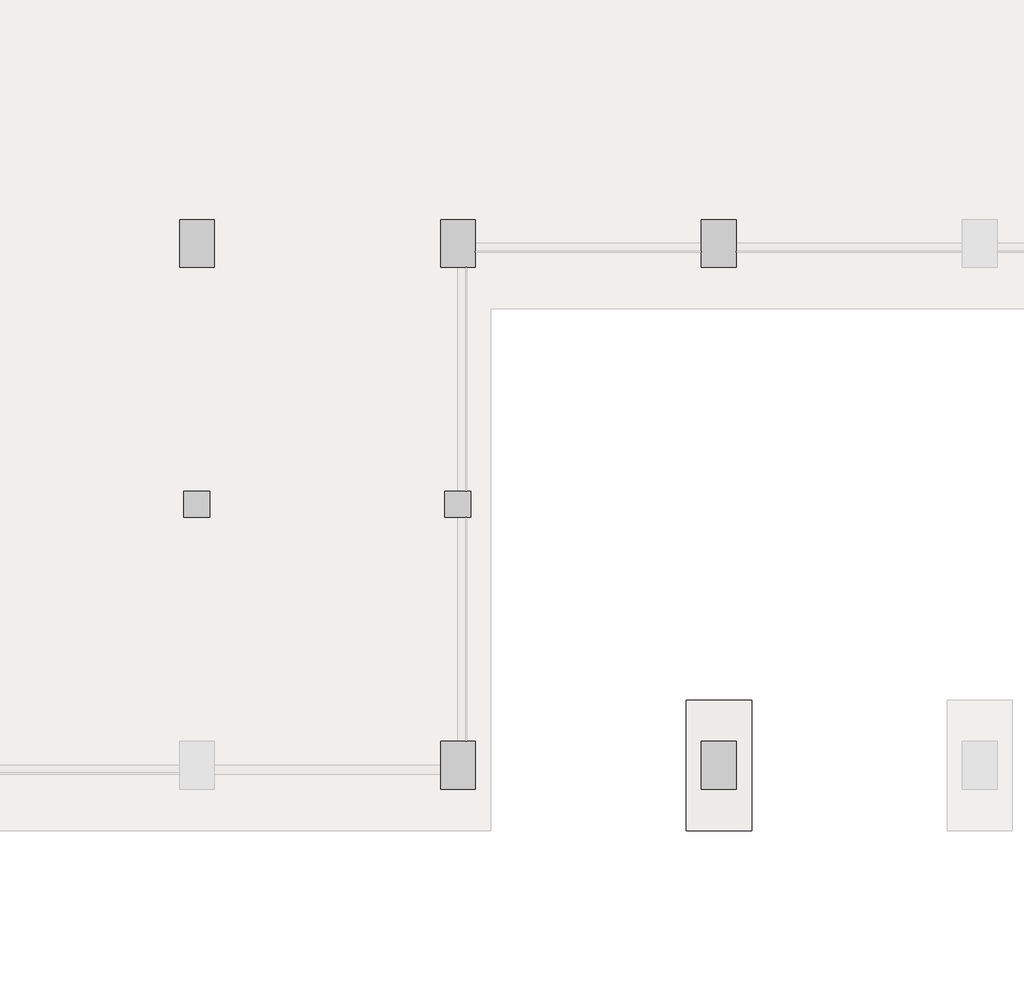
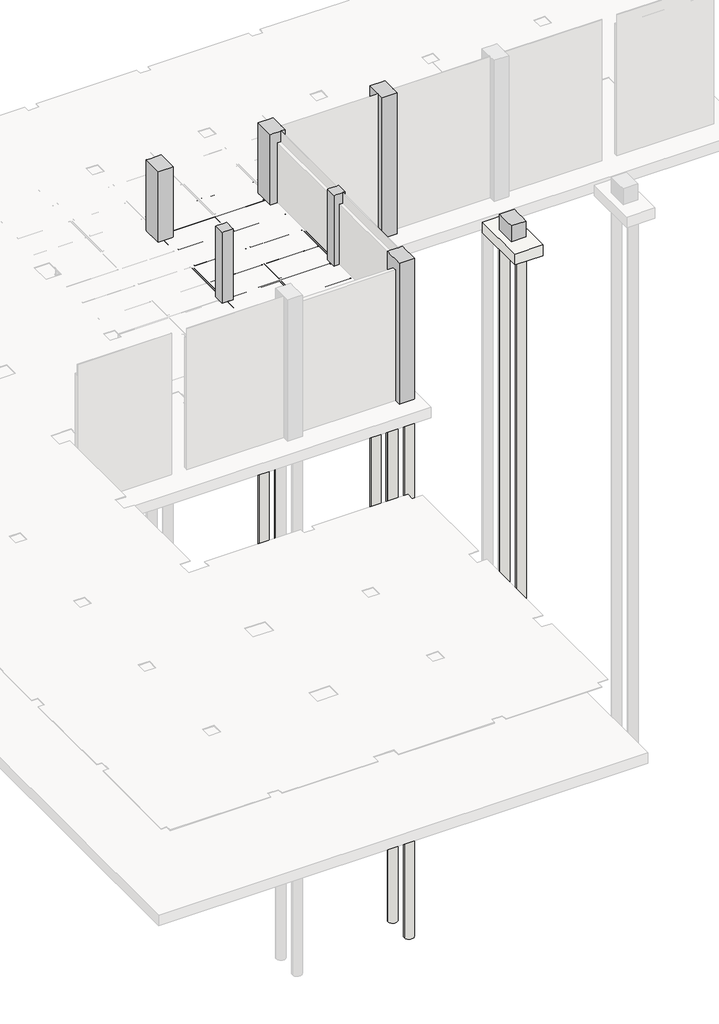
# Not in any storey, part 11 of 16: 24 beams, 9 slabs, 7 columns.
"""IFC4 building model written with IfcOpenShell, lengths in millimetres."""

from ifc_helpers import new_model, si_unit, point, frame, frame_2d, origin, place, context, project, spatial, polyline, circle_curve, trimmed, segment, composite_curve, outline, extrude, faceted_brep, element, save

model = new_model("IFC4")

# Units and contexts
model_context = context("Model", 3, world=origin())
ifc_project = project(units=[si_unit("LENGTHUNIT", "METRE", prefix="MILLI")], contexts=[model_context])

# Site, building
site = spatial("IfcSite", under=ifc_project)
building = spatial("IfcBuilding", under=site)

# Beams
placement = place(None, origin())
element("IfcBeam", 1, ObjectType="Steel Framing_H_KS : H_SB_AR_S02_H-400x200x8x13_BSG1", at=placement, inside=building, context=model_context, shape_type="SweptSolid", body=[
    extrude(outline(composite_curve([segment(polyline([(-17900.0, -4187.0381366), (-17900.0, -4200.0381366), (-18100.0, -4200.0381366), (-18100.0, -4187.0381366), (-18020.0, -4187.0381366)]), True, "CONTINUOUS"), segment(trimmed(circle_curve(frame_2d((-18020.0, -4171.0381366)), 16.0), [point((-18020.0, -4187.0381366))], [point((-18004.0, -4171.0381366))], True, "CARTESIAN"), True, "CONTINUOUS"), segment(polyline([(-18004.0, -4171.0381366), (-18004.0, -3829.0381366)]), True, "CONTINUOUS"), segment(trimmed(circle_curve(frame_2d((-18020.0, -3829.0381366)), 16.0), [point((-18004.0, -3829.0381366))], [point((-18020.0, -3813.0381366))], True, "CARTESIAN"), True, "CONTINUOUS"), segment(polyline([(-18020.0, -3813.0381366), (-18100.0, -3813.0381366), (-18100.0, -3800.0381366), (-17900.0, -3800.0381366), (-17900.0, -3813.0381366), (-17980.0, -3813.0381366)]), True, "CONTINUOUS"), segment(trimmed(circle_curve(frame_2d((-17980.0, -3829.0381366)), 16.0), [point((-17980.0, -3813.0381366))], [point((-17996.0, -3829.0381366))], True, "CARTESIAN"), True, "CONTINUOUS"), segment(polyline([(-17996.0, -3829.0381366), (-17996.0, -4171.0381366)]), True, "CONTINUOUS"), segment(trimmed(circle_curve(frame_2d((-17980.0, -4171.0381366)), 16.0), [point((-17996.0, -4171.0381366))], [point((-17980.0, -4187.0381366))], True, "CARTESIAN"), True, "CONTINUOUS"), segment(polyline([(-17980.0, -4187.0381366), (-17900.0, -4187.0381366)]), True, "CONTINUOUS")], self_intersect=False)), frame((48412.7, 0.0, 0.0), z_axis=(1.0, 0.0, 0.0), x_axis=(0.0, 1.0, 0.0)), (0.0, 0.0, 1.0), 5174.6),
])
element("IfcBeam", 2, ObjectType="Steel Framing_C_KS : H_SB_AR_S02_C-150x75x6.5x10_J1", at=placement, inside=building, context=model_context, shape_type="SweptSolid", body=[
    extrude(outline(composite_curve([segment(polyline([(-16477.2, -3800.0381366), (-16477.2, -3950.0381366), (-16552.2, -3950.0381366)]), True, "CONTINUOUS"), segment(trimmed(circle_curve(frame_2d((-16542.2, -3950.0381366)), 10.0), [point((-16552.2, -3950.0381366))], [point((-16542.2, -3940.0381366))], False, "CARTESIAN"), True, "CONTINUOUS"), segment(polyline([(-16542.2, -3940.0381366), (-16483.7, -3930.7726469), (-16483.7, -3819.3036264), (-16542.2, -3810.0381366)]), True, "CONTINUOUS"), segment(trimmed(circle_curve(frame_2d((-16542.2, -3800.0381366)), 10.0), [point((-16542.2, -3810.0381366))], [point((-16552.2, -3800.0381366))], False, "CARTESIAN"), True, "CONTINUOUS"), segment(polyline([(-16552.2, -3800.0381366), (-16477.2, -3800.0381366)]), True, "CONTINUOUS")], self_intersect=False)), frame((48112.7, 0.0, 0.0), z_axis=(1.0, 0.0, 0.0), x_axis=(0.0, 1.0, 0.0)), (0.0, 0.0, 1.0), 2774.6),
])
element("IfcBeam", 3, ObjectType="Steel Framing_C_KS : H_SB_AR_S02_C-150x75x6.5x10_J1", at=placement, inside=building, context=model_context, shape_type="SweptSolid", body=[
    extrude(outline(composite_curve([segment(polyline([(-16477.2, -3800.0381366), (-16477.2, -3950.0381366), (-16552.2, -3950.0381366)]), True, "CONTINUOUS"), segment(trimmed(circle_curve(frame_2d((-16542.2, -3950.0381366)), 10.0), [point((-16552.2, -3950.0381366))], [point((-16542.2, -3940.0381366))], False, "CARTESIAN"), True, "CONTINUOUS"), segment(polyline([(-16542.2, -3940.0381366), (-16483.7, -3930.7726469), (-16483.7, -3819.3036264), (-16542.2, -3810.0381366)]), True, "CONTINUOUS"), segment(trimmed(circle_curve(frame_2d((-16542.2, -3800.0381366)), 10.0), [point((-16542.2, -3810.0381366))], [point((-16552.2, -3800.0381366))], False, "CARTESIAN"), True, "CONTINUOUS"), segment(polyline([(-16552.2, -3800.0381366), (-16477.2, -3800.0381366)]), True, "CONTINUOUS")], self_intersect=False)), frame((51112.7, 0.0, 0.0), z_axis=(1.0, 0.0, 0.0), x_axis=(0.0, 1.0, 0.0)), (0.0, 0.0, 1.0), 2774.6),
])
element("IfcBeam", 4, ObjectType="Steel Framing_C_KS : H_SB_AR_S02_C-150x75x6.5x10_J1", at=placement, inside=building, context=model_context, shape_type="SweptSolid", body=[
    extrude(outline(composite_curve([segment(polyline([(-16477.2, -3800.0381366), (-16477.2, -3950.0381366), (-16552.2, -3950.0381366)]), True, "CONTINUOUS"), segment(trimmed(circle_curve(frame_2d((-16542.2, -3950.0381366)), 10.0), [point((-16552.2, -3950.0381366))], [point((-16542.2, -3940.0381366))], False, "CARTESIAN"), True, "CONTINUOUS"), segment(polyline([(-16542.2, -3940.0381366), (-16483.7, -3930.7726469), (-16483.7, -3819.3036264), (-16542.2, -3810.0381366)]), True, "CONTINUOUS"), segment(trimmed(circle_curve(frame_2d((-16542.2, -3800.0381366)), 10.0), [point((-16542.2, -3810.0381366))], [point((-16552.2, -3800.0381366))], False, "CARTESIAN"), True, "CONTINUOUS"), segment(polyline([(-16552.2, -3800.0381366), (-16477.2, -3800.0381366)]), True, "CONTINUOUS")], self_intersect=False)), frame((54112.7, 0.0, 0.0), z_axis=(1.0, 0.0, 0.0), x_axis=(0.0, 1.0, 0.0)), (0.0, 0.0, 1.0), 2774.6),
])
element("IfcBeam", 5, ObjectType="Steel Framing_C_KS : H_SB_AR_S02_C-150x75x6.5x10_J1", at=placement, inside=building, context=model_context, shape_type="SweptSolid", body=[
    extrude(outline(composite_curve([segment(polyline([(-16477.2, -3800.0381366), (-16477.2, -3950.0381366), (-16552.2, -3950.0381366)]), True, "CONTINUOUS"), segment(trimmed(circle_curve(frame_2d((-16542.2, -3950.0381366)), 10.0), [point((-16552.2, -3950.0381366))], [point((-16542.2, -3940.0381366))], False, "CARTESIAN"), True, "CONTINUOUS"), segment(polyline([(-16542.2, -3940.0381366), (-16483.7, -3930.7726469), (-16483.7, -3819.3036264), (-16542.2, -3810.0381366)]), True, "CONTINUOUS"), segment(trimmed(circle_curve(frame_2d((-16542.2, -3800.0381366)), 10.0), [point((-16542.2, -3810.0381366))], [point((-16552.2, -3800.0381366))], False, "CARTESIAN"), True, "CONTINUOUS"), segment(polyline([(-16552.2, -3800.0381366), (-16477.2, -3800.0381366)]), True, "CONTINUOUS")], self_intersect=False)), frame((57112.7, 0.0, 0.0), z_axis=(1.0, 0.0, 0.0), x_axis=(0.0, 1.0, 0.0)), (0.0, 0.0, 1.0), 2774.6),
])
element("IfcBeam", 6, ObjectType="Steel Framing_C_KS : H_SB_AR_S02_C-150x75x6.5x10_J1", at=placement, inside=building, context=model_context, shape_type="SweptSolid", body=[
    extrude(outline(composite_curve([segment(polyline([(-16477.2, -3800.0381366), (-16477.2, -3950.0381366), (-16552.2, -3950.0381366)]), True, "CONTINUOUS"), segment(trimmed(circle_curve(frame_2d((-16542.2, -3950.0381366)), 10.0), [point((-16552.2, -3950.0381366))], [point((-16542.2, -3940.0381366))], False, "CARTESIAN"), True, "CONTINUOUS"), segment(polyline([(-16542.2, -3940.0381366), (-16483.7, -3930.7726469), (-16483.7, -3819.3036264), (-16542.2, -3810.0381366)]), True, "CONTINUOUS"), segment(trimmed(circle_curve(frame_2d((-16542.2, -3800.0381366)), 10.0), [point((-16542.2, -3810.0381366))], [point((-16552.2, -3800.0381366))], False, "CARTESIAN"), True, "CONTINUOUS"), segment(polyline([(-16552.2, -3800.0381366), (-16477.2, -3800.0381366)]), True, "CONTINUOUS")], self_intersect=False)), frame((60112.7, 0.0, 0.0), z_axis=(1.0, 0.0, 0.0), x_axis=(0.0, 1.0, 0.0)), (0.0, 0.0, 1.0), 2774.6),
])
element("IfcBeam", 7, ObjectType="Steel Framing_H_KS : H_SB_AR_S02_H-400x200x8x13_BSG2", at=placement, inside=building, context=model_context, shape_type="SweptSolid", body=[
    extrude(outline(composite_curve([segment(polyline([(-4187.0381366, 47900.0), (-4200.0381366, 47900.0), (-4200.0381366, 48100.0), (-4187.0381366, 48100.0), (-4187.0381366, 48020.0)]), True, "CONTINUOUS"), segment(trimmed(circle_curve(frame_2d((-4171.0381366, 48020.0)), 16.0), [point((-4187.0381366, 48020.0))], [point((-4171.0381366, 48004.0))], True, "CARTESIAN"), True, "CONTINUOUS"), segment(polyline([(-4171.0381366, 48004.0), (-3829.0381366, 48004.0)]), True, "CONTINUOUS"), segment(trimmed(circle_curve(frame_2d((-3829.0381366, 48020.0)), 16.0), [point((-3829.0381366, 48004.0))], [point((-3813.0381366, 48020.0))], True, "CARTESIAN"), True, "CONTINUOUS"), segment(polyline([(-3813.0381366, 48020.0), (-3813.0381366, 48100.0), (-3800.0381366, 48100.0), (-3800.0381366, 47900.0), (-3813.0381366, 47900.0), (-3813.0381366, 47980.0)]), True, "CONTINUOUS"), segment(trimmed(circle_curve(frame_2d((-3829.0381366, 47980.0)), 16.0), [point((-3813.0381366, 47980.0))], [point((-3829.0381366, 47996.0))], True, "CARTESIAN"), True, "CONTINUOUS"), segment(polyline([(-3829.0381366, 47996.0), (-4171.0381366, 47996.0)]), True, "CONTINUOUS"), segment(trimmed(circle_curve(frame_2d((-4171.0381366, 47980.0)), 16.0), [point((-4171.0381366, 47996.0))], [point((-4187.0381366, 47980.0))], True, "CARTESIAN"), True, "CONTINUOUS"), segment(polyline([(-4187.0381366, 47980.0), (-4187.0381366, 47900.0)]), True, "CONTINUOUS")], self_intersect=False)), frame((0.0, -23687.3, 0.0), z_axis=(0.0, 1.0, 0.0), x_axis=(0.0, 0.0, 1.0)), (0.0, 0.0, 1.0), 5124.6),
])
element("IfcBeam", 8, ObjectType="Steel Framing_H_KS : H_SB_AR_S02_H-400x200x8x13_BSG1", at=placement, inside=building, context=model_context, shape_type="SweptSolid", body=[
    extrude(outline(composite_curve([segment(polyline([(-23900.0, -4187.0381366), (-23900.0, -4200.0381366), (-24100.0, -4200.0381366), (-24100.0, -4187.0381366), (-24020.0, -4187.0381366)]), True, "CONTINUOUS"), segment(trimmed(circle_curve(frame_2d((-24020.0, -4171.0381366)), 16.0), [point((-24020.0, -4187.0381366))], [point((-24004.0, -4171.0381366))], True, "CARTESIAN"), True, "CONTINUOUS"), segment(polyline([(-24004.0, -4171.0381366), (-24004.0, -3829.0381366)]), True, "CONTINUOUS"), segment(trimmed(circle_curve(frame_2d((-24020.0, -3829.0381366)), 16.0), [point((-24004.0, -3829.0381366))], [point((-24020.0, -3813.0381366))], True, "CARTESIAN"), True, "CONTINUOUS"), segment(polyline([(-24020.0, -3813.0381366), (-24100.0, -3813.0381366), (-24100.0, -3800.0381366), (-23900.0, -3800.0381366), (-23900.0, -3813.0381366), (-23980.0, -3813.0381366)]), True, "CONTINUOUS"), segment(trimmed(circle_curve(frame_2d((-23980.0, -3829.0381366)), 16.0), [point((-23980.0, -3813.0381366))], [point((-23996.0, -3829.0381366))], True, "CARTESIAN"), True, "CONTINUOUS"), segment(polyline([(-23996.0, -3829.0381366), (-23996.0, -4171.0381366)]), True, "CONTINUOUS"), segment(trimmed(circle_curve(frame_2d((-23980.0, -4171.0381366)), 16.0), [point((-23996.0, -4171.0381366))], [point((-23980.0, -4187.0381366))], True, "CARTESIAN"), True, "CONTINUOUS"), segment(polyline([(-23980.0, -4187.0381366), (-23900.0, -4187.0381366)]), True, "CONTINUOUS")], self_intersect=False)), frame((48312.7, 0.0, 0.0), z_axis=(1.0, 0.0, 0.0), x_axis=(0.0, 1.0, 0.0)), (0.0, 0.0, 1.0), 5374.6),
])
element("IfcBeam", 9, ObjectType="Steel Framing_H_KS : H_SB_AR_S02_H-400x200x8x13_BSG2", at=placement, inside=building, context=model_context, shape_type="SweptSolid", body=[
    extrude(outline(composite_curve([segment(polyline([(-4187.0381366, 53900.0), (-4200.0381366, 53900.0), (-4200.0381366, 54100.0), (-4187.0381366, 54100.0), (-4187.0381366, 54020.0)]), True, "CONTINUOUS"), segment(trimmed(circle_curve(frame_2d((-4171.0381366, 54020.0)), 16.0), [point((-4187.0381366, 54020.0))], [point((-4171.0381366, 54004.0))], True, "CARTESIAN"), True, "CONTINUOUS"), segment(polyline([(-4171.0381366, 54004.0), (-3829.0381366, 54004.0)]), True, "CONTINUOUS"), segment(trimmed(circle_curve(frame_2d((-3829.0381366, 54020.0)), 16.0), [point((-3829.0381366, 54004.0))], [point((-3813.0381366, 54020.0))], True, "CARTESIAN"), True, "CONTINUOUS"), segment(polyline([(-3813.0381366, 54020.0), (-3813.0381366, 54100.0), (-3800.0381366, 54100.0), (-3800.0381366, 53900.0), (-3813.0381366, 53900.0), (-3813.0381366, 53980.0)]), True, "CONTINUOUS"), segment(trimmed(circle_curve(frame_2d((-3829.0381366, 53980.0)), 16.0), [point((-3813.0381366, 53980.0))], [point((-3829.0381366, 53996.0))], True, "CARTESIAN"), True, "CONTINUOUS"), segment(polyline([(-3829.0381366, 53996.0), (-4171.0381366, 53996.0)]), True, "CONTINUOUS"), segment(trimmed(circle_curve(frame_2d((-4171.0381366, 53980.0)), 16.0), [point((-4171.0381366, 53996.0))], [point((-4187.0381366, 53980.0))], True, "CARTESIAN"), True, "CONTINUOUS"), segment(polyline([(-4187.0381366, 53980.0), (-4187.0381366, 53900.0)]), True, "CONTINUOUS")], self_intersect=False)), frame((0.0, -23687.3, 0.0), z_axis=(0.0, 1.0, 0.0), x_axis=(0.0, 0.0, 1.0)), (0.0, 0.0, 1.0), 5124.6),
])
element("IfcBeam", 10, ObjectType="Steel Framing_H_KS : H_SB_AR_S02_H-400x200x8x13_BSB1", at=placement, inside=building, context=model_context, shape_type="SweptSolid", body=[
    extrude(outline(composite_curve([segment(polyline([(-4187.0381366, 50900.0), (-4200.0381366, 50900.0), (-4200.0381366, 51100.0), (-4187.0381366, 51100.0), (-4187.0381366, 51020.0)]), True, "CONTINUOUS"), segment(trimmed(circle_curve(frame_2d((-4171.0381366, 51020.0)), 16.0), [point((-4187.0381366, 51020.0))], [point((-4171.0381366, 51004.0))], True, "CARTESIAN"), True, "CONTINUOUS"), segment(polyline([(-4171.0381366, 51004.0), (-3829.0381366, 51004.0)]), True, "CONTINUOUS"), segment(trimmed(circle_curve(frame_2d((-3829.0381366, 51020.0)), 16.0), [point((-3829.0381366, 51004.0))], [point((-3813.0381366, 51020.0))], True, "CARTESIAN"), True, "CONTINUOUS"), segment(polyline([(-3813.0381366, 51020.0), (-3813.0381366, 51100.0), (-3800.0381366, 51100.0), (-3800.0381366, 50900.0), (-3813.0381366, 50900.0), (-3813.0381366, 50980.0)]), True, "CONTINUOUS"), segment(trimmed(circle_curve(frame_2d((-3829.0381366, 50980.0)), 16.0), [point((-3813.0381366, 50980.0))], [point((-3829.0381366, 50996.0))], True, "CARTESIAN"), True, "CONTINUOUS"), segment(polyline([(-3829.0381366, 50996.0), (-4171.0381366, 50996.0)]), True, "CONTINUOUS"), segment(trimmed(circle_curve(frame_2d((-4171.0381366, 50980.0)), 16.0), [point((-4171.0381366, 50996.0))], [point((-4187.0381366, 50980.0))], True, "CARTESIAN"), True, "CONTINUOUS"), segment(polyline([(-4187.0381366, 50980.0), (-4187.0381366, 50900.0)]), True, "CONTINUOUS")], self_intersect=False)), frame((0.0, -23887.3, 0.0), z_axis=(0.0, 1.0, 0.0), x_axis=(0.0, 0.0, 1.0)), (0.0, 0.0, 1.0), 5774.6),
])
element("IfcBeam", 11, ObjectType="Steel Framing_C_KS : H_SB_AR_S02_C-150x75x6.5x10_J1", at=placement, inside=building, context=model_context, shape_type="SweptSolid", body=[
    extrude(outline(composite_curve([segment(polyline([(-20977.2, -3800.0381366), (-20977.2, -3950.0381366), (-21052.2, -3950.0381366)]), True, "CONTINUOUS"), segment(trimmed(circle_curve(frame_2d((-21042.2, -3950.0381366)), 10.0), [point((-21052.2, -3950.0381366))], [point((-21042.2, -3940.0381366))], False, "CARTESIAN"), True, "CONTINUOUS"), segment(polyline([(-21042.2, -3940.0381366), (-20983.7, -3930.7726469), (-20983.7, -3819.3036264), (-21042.2, -3810.0381366)]), True, "CONTINUOUS"), segment(trimmed(circle_curve(frame_2d((-21042.2, -3800.0381366)), 10.0), [point((-21042.2, -3810.0381366))], [point((-21052.2, -3800.0381366))], False, "CARTESIAN"), True, "CONTINUOUS"), segment(polyline([(-21052.2, -3800.0381366), (-20977.2, -3800.0381366)]), True, "CONTINUOUS")], self_intersect=False)), frame((48112.7, 0.0, 0.0), z_axis=(1.0, 0.0, 0.0), x_axis=(0.0, 1.0, 0.0)), (0.0, 0.0, 1.0), 2774.6),
])
element("IfcBeam", 12, ObjectType="Steel Framing_C_KS : H_SB_AR_S02_C-150x75x6.5x10_J1", at=placement, inside=building, context=model_context, shape_type="SweptSolid", body=[
    extrude(outline(composite_curve([segment(polyline([(-22477.2, -3800.0381366), (-22477.2, -3950.0381366), (-22552.2, -3950.0381366)]), True, "CONTINUOUS"), segment(trimmed(circle_curve(frame_2d((-22542.2, -3950.0381366)), 10.0), [point((-22552.2, -3950.0381366))], [point((-22542.2, -3940.0381366))], False, "CARTESIAN"), True, "CONTINUOUS"), segment(polyline([(-22542.2, -3940.0381366), (-22483.7, -3930.7726469), (-22483.7, -3819.3036264), (-22542.2, -3810.0381366)]), True, "CONTINUOUS"), segment(trimmed(circle_curve(frame_2d((-22542.2, -3800.0381366)), 10.0), [point((-22542.2, -3810.0381366))], [point((-22552.2, -3800.0381366))], False, "CARTESIAN"), True, "CONTINUOUS"), segment(polyline([(-22552.2, -3800.0381366), (-22477.2, -3800.0381366)]), True, "CONTINUOUS")], self_intersect=False)), frame((48112.7, 0.0, 0.0), z_axis=(1.0, 0.0, 0.0), x_axis=(0.0, 1.0, 0.0)), (0.0, 0.0, 1.0), 2774.6),
])
element("IfcBeam", 13, ObjectType="Steel Framing_C_KS : H_SB_AR_S02_C-150x75x6.5x10_J1", at=placement, inside=building, context=model_context, shape_type="SweptSolid", body=[
    extrude(outline(composite_curve([segment(polyline([(-19477.2, -3800.0381366), (-19477.2, -3950.0381366), (-19552.2, -3950.0381366)]), True, "CONTINUOUS"), segment(trimmed(circle_curve(frame_2d((-19542.2, -3950.0381366)), 10.0), [point((-19552.2, -3950.0381366))], [point((-19542.2, -3940.0381366))], False, "CARTESIAN"), True, "CONTINUOUS"), segment(polyline([(-19542.2, -3940.0381366), (-19483.7, -3930.7726469), (-19483.7, -3819.3036264), (-19542.2, -3810.0381366)]), True, "CONTINUOUS"), segment(trimmed(circle_curve(frame_2d((-19542.2, -3800.0381366)), 10.0), [point((-19542.2, -3810.0381366))], [point((-19552.2, -3800.0381366))], False, "CARTESIAN"), True, "CONTINUOUS"), segment(polyline([(-19552.2, -3800.0381366), (-19477.2, -3800.0381366)]), True, "CONTINUOUS")], self_intersect=False)), frame((48112.7, 0.0, 0.0), z_axis=(1.0, 0.0, 0.0), x_axis=(0.0, 1.0, 0.0)), (0.0, 0.0, 1.0), 2774.6),
])
element("IfcBeam", 14, ObjectType="Steel Framing_C_KS : H_SB_AR_S02_C-150x75x6.5x10_J1", at=placement, inside=building, context=model_context, shape_type="SweptSolid", body=[
    extrude(outline(composite_curve([segment(polyline([(-20977.2, -3800.0381366), (-20977.2, -3950.0381366), (-21052.2, -3950.0381366)]), True, "CONTINUOUS"), segment(trimmed(circle_curve(frame_2d((-21042.2, -3950.0381366)), 10.0), [point((-21052.2, -3950.0381366))], [point((-21042.2, -3940.0381366))], False, "CARTESIAN"), True, "CONTINUOUS"), segment(polyline([(-21042.2, -3940.0381366), (-20983.7, -3930.7726469), (-20983.7, -3819.3036264), (-21042.2, -3810.0381366)]), True, "CONTINUOUS"), segment(trimmed(circle_curve(frame_2d((-21042.2, -3800.0381366)), 10.0), [point((-21042.2, -3810.0381366))], [point((-21052.2, -3800.0381366))], False, "CARTESIAN"), True, "CONTINUOUS"), segment(polyline([(-21052.2, -3800.0381366), (-20977.2, -3800.0381366)]), True, "CONTINUOUS")], self_intersect=False)), frame((51112.7, 0.0, 0.0), z_axis=(1.0, 0.0, 0.0), x_axis=(0.0, 1.0, 0.0)), (0.0, 0.0, 1.0), 2774.6),
])
element("IfcBeam", 15, ObjectType="Steel Framing_C_KS : H_SB_AR_S02_C-150x75x6.5x10_J1", at=placement, inside=building, context=model_context, shape_type="SweptSolid", body=[
    extrude(outline(composite_curve([segment(polyline([(-22477.2, -3800.0381366), (-22477.2, -3950.0381366), (-22552.2, -3950.0381366)]), True, "CONTINUOUS"), segment(trimmed(circle_curve(frame_2d((-22542.2, -3950.0381366)), 10.0), [point((-22552.2, -3950.0381366))], [point((-22542.2, -3940.0381366))], False, "CARTESIAN"), True, "CONTINUOUS"), segment(polyline([(-22542.2, -3940.0381366), (-22483.7, -3930.7726469), (-22483.7, -3819.3036264), (-22542.2, -3810.0381366)]), True, "CONTINUOUS"), segment(trimmed(circle_curve(frame_2d((-22542.2, -3800.0381366)), 10.0), [point((-22542.2, -3810.0381366))], [point((-22552.2, -3800.0381366))], False, "CARTESIAN"), True, "CONTINUOUS"), segment(polyline([(-22552.2, -3800.0381366), (-22477.2, -3800.0381366)]), True, "CONTINUOUS")], self_intersect=False)), frame((51112.7, 0.0, 0.0), z_axis=(1.0, 0.0, 0.0), x_axis=(0.0, 1.0, 0.0)), (0.0, 0.0, 1.0), 2774.6),
])
element("IfcBeam", 16, ObjectType="Steel Framing_C_KS : H_SB_AR_S02_C-150x75x6.5x10_J1", at=placement, inside=building, context=model_context, shape_type="SweptSolid", body=[
    extrude(outline(composite_curve([segment(polyline([(-19477.2, -3800.0381366), (-19477.2, -3950.0381366), (-19552.2, -3950.0381366)]), True, "CONTINUOUS"), segment(trimmed(circle_curve(frame_2d((-19542.2, -3950.0381366)), 10.0), [point((-19552.2, -3950.0381366))], [point((-19542.2, -3940.0381366))], False, "CARTESIAN"), True, "CONTINUOUS"), segment(polyline([(-19542.2, -3940.0381366), (-19483.7, -3930.7726469), (-19483.7, -3819.3036264), (-19542.2, -3810.0381366)]), True, "CONTINUOUS"), segment(trimmed(circle_curve(frame_2d((-19542.2, -3800.0381366)), 10.0), [point((-19542.2, -3810.0381366))], [point((-19552.2, -3800.0381366))], False, "CARTESIAN"), True, "CONTINUOUS"), segment(polyline([(-19552.2, -3800.0381366), (-19477.2, -3800.0381366)]), True, "CONTINUOUS")], self_intersect=False)), frame((51112.7, 0.0, 0.0), z_axis=(1.0, 0.0, 0.0), x_axis=(0.0, 1.0, 0.0)), (0.0, 0.0, 1.0), 2774.6),
])
element("IfcBeam", 17, ObjectType="Steel Framing_H_KS : H_SB_AR_S02_H-400x200x8x13_BSG2", at=placement, inside=building, context=model_context, shape_type="SweptSolid", body=[
    extrude(outline(composite_curve([segment(polyline([(-4187.0381366, 47900.0), (-4200.0381366, 47900.0), (-4200.0381366, 48100.0), (-4187.0381366, 48100.0), (-4187.0381366, 48020.0)]), True, "CONTINUOUS"), segment(trimmed(circle_curve(frame_2d((-4171.0381366, 48020.0)), 16.0), [point((-4187.0381366, 48020.0))], [point((-4171.0381366, 48004.0))], True, "CARTESIAN"), True, "CONTINUOUS"), segment(polyline([(-4171.0381366, 48004.0), (-3829.0381366, 48004.0)]), True, "CONTINUOUS"), segment(trimmed(circle_curve(frame_2d((-3829.0381366, 48020.0)), 16.0), [point((-3829.0381366, 48004.0))], [point((-3813.0381366, 48020.0))], True, "CARTESIAN"), True, "CONTINUOUS"), segment(polyline([(-3813.0381366, 48020.0), (-3813.0381366, 48100.0), (-3800.0381366, 48100.0), (-3800.0381366, 47900.0), (-3813.0381366, 47900.0), (-3813.0381366, 47980.0)]), True, "CONTINUOUS"), segment(trimmed(circle_curve(frame_2d((-3829.0381366, 47980.0)), 16.0), [point((-3813.0381366, 47980.0))], [point((-3829.0381366, 47996.0))], True, "CARTESIAN"), True, "CONTINUOUS"), segment(polyline([(-3829.0381366, 47996.0), (-4171.0381366, 47996.0)]), True, "CONTINUOUS"), segment(trimmed(circle_curve(frame_2d((-4171.0381366, 47980.0)), 16.0), [point((-4171.0381366, 47996.0))], [point((-4187.0381366, 47980.0))], True, "CARTESIAN"), True, "CONTINUOUS"), segment(polyline([(-4187.0381366, 47980.0), (-4187.0381366, 47900.0)]), True, "CONTINUOUS")], self_intersect=False)), frame((0.0, -29437.3, 0.0), z_axis=(0.0, 1.0, 0.0), x_axis=(0.0, 0.0, 1.0)), (0.0, 0.0, 1.0), 5124.6),
])
element("IfcBeam", 18, ObjectType="Steel Framing_H_KS : H_SB_AR_S02_H-400x200x8x13_BSG2", at=placement, inside=building, context=model_context, shape_type="SweptSolid", body=[
    extrude(outline(composite_curve([segment(polyline([(-4187.0381366, 53900.0), (-4200.0381366, 53900.0), (-4200.0381366, 54100.0), (-4187.0381366, 54100.0), (-4187.0381366, 54020.0)]), True, "CONTINUOUS"), segment(trimmed(circle_curve(frame_2d((-4171.0381366, 54020.0)), 16.0), [point((-4187.0381366, 54020.0))], [point((-4171.0381366, 54004.0))], True, "CARTESIAN"), True, "CONTINUOUS"), segment(polyline([(-4171.0381366, 54004.0), (-3829.0381366, 54004.0)]), True, "CONTINUOUS"), segment(trimmed(circle_curve(frame_2d((-3829.0381366, 54020.0)), 16.0), [point((-3829.0381366, 54004.0))], [point((-3813.0381366, 54020.0))], True, "CARTESIAN"), True, "CONTINUOUS"), segment(polyline([(-3813.0381366, 54020.0), (-3813.0381366, 54100.0), (-3800.0381366, 54100.0), (-3800.0381366, 53900.0), (-3813.0381366, 53900.0), (-3813.0381366, 53980.0)]), True, "CONTINUOUS"), segment(trimmed(circle_curve(frame_2d((-3829.0381366, 53980.0)), 16.0), [point((-3813.0381366, 53980.0))], [point((-3829.0381366, 53996.0))], True, "CARTESIAN"), True, "CONTINUOUS"), segment(polyline([(-3829.0381366, 53996.0), (-4171.0381366, 53996.0)]), True, "CONTINUOUS"), segment(trimmed(circle_curve(frame_2d((-4171.0381366, 53980.0)), 16.0), [point((-4171.0381366, 53996.0))], [point((-4187.0381366, 53980.0))], True, "CARTESIAN"), True, "CONTINUOUS"), segment(polyline([(-4187.0381366, 53980.0), (-4187.0381366, 53900.0)]), True, "CONTINUOUS")], self_intersect=False)), frame((0.0, -29437.3, 0.0), z_axis=(0.0, 1.0, 0.0), x_axis=(0.0, 0.0, 1.0)), (0.0, 0.0, 1.0), 5124.6),
])
element("IfcBeam", 19, ObjectType="Steel Framing_H_KS : H_SB_AR_S02_H-400x200x8x13_BSB1", at=placement, inside=building, context=model_context, shape_type="SweptSolid", body=[
    extrude(outline(composite_curve([segment(polyline([(-4187.0381366, 50900.0), (-4200.0381366, 50900.0), (-4200.0381366, 51100.0), (-4187.0381366, 51100.0), (-4187.0381366, 51020.0)]), True, "CONTINUOUS"), segment(trimmed(circle_curve(frame_2d((-4171.0381366, 51020.0)), 16.0), [point((-4187.0381366, 51020.0))], [point((-4171.0381366, 51004.0))], True, "CARTESIAN"), True, "CONTINUOUS"), segment(polyline([(-4171.0381366, 51004.0), (-3829.0381366, 51004.0)]), True, "CONTINUOUS"), segment(trimmed(circle_curve(frame_2d((-3829.0381366, 51020.0)), 16.0), [point((-3829.0381366, 51004.0))], [point((-3813.0381366, 51020.0))], True, "CARTESIAN"), True, "CONTINUOUS"), segment(polyline([(-3813.0381366, 51020.0), (-3813.0381366, 51100.0), (-3800.0381366, 51100.0), (-3800.0381366, 50900.0), (-3813.0381366, 50900.0), (-3813.0381366, 50980.0)]), True, "CONTINUOUS"), segment(trimmed(circle_curve(frame_2d((-3829.0381366, 50980.0)), 16.0), [point((-3813.0381366, 50980.0))], [point((-3829.0381366, 50996.0))], True, "CARTESIAN"), True, "CONTINUOUS"), segment(polyline([(-3829.0381366, 50996.0), (-4171.0381366, 50996.0)]), True, "CONTINUOUS"), segment(trimmed(circle_curve(frame_2d((-4171.0381366, 50980.0)), 16.0), [point((-4171.0381366, 50996.0))], [point((-4187.0381366, 50980.0))], True, "CARTESIAN"), True, "CONTINUOUS"), segment(polyline([(-4187.0381366, 50980.0), (-4187.0381366, 50900.0)]), True, "CONTINUOUS")], self_intersect=False)), frame((0.0, -29887.3, 0.0), z_axis=(0.0, 1.0, 0.0), x_axis=(0.0, 0.0, 1.0)), (0.0, 0.0, 1.0), 5774.6),
])
element("IfcBeam", 20, ObjectType="Steel Framing_C_KS : H_SB_AR_S02_C-150x75x6.5x10_J1", at=placement, inside=building, context=model_context, shape_type="SweptSolid", body=[
    extrude(outline(composite_curve([segment(polyline([(-26977.2, -3800.0381366), (-26977.2, -3950.0381366), (-27052.2, -3950.0381366)]), True, "CONTINUOUS"), segment(trimmed(circle_curve(frame_2d((-27042.2, -3950.0381366)), 10.0), [point((-27052.2, -3950.0381366))], [point((-27042.2, -3940.0381366))], False, "CARTESIAN"), True, "CONTINUOUS"), segment(polyline([(-27042.2, -3940.0381366), (-26983.7, -3930.7726469), (-26983.7, -3819.3036264), (-27042.2, -3810.0381366)]), True, "CONTINUOUS"), segment(trimmed(circle_curve(frame_2d((-27042.2, -3800.0381366)), 10.0), [point((-27042.2, -3810.0381366))], [point((-27052.2, -3800.0381366))], False, "CARTESIAN"), True, "CONTINUOUS"), segment(polyline([(-27052.2, -3800.0381366), (-26977.2, -3800.0381366)]), True, "CONTINUOUS")], self_intersect=False)), frame((48112.7, 0.0, 0.0), z_axis=(1.0, 0.0, 0.0), x_axis=(0.0, 1.0, 0.0)), (0.0, 0.0, 1.0), 2774.6),
])
element("IfcBeam", 21, ObjectType="Steel Framing_C_KS : H_SB_AR_S02_C-150x75x6.5x10_J1", at=placement, inside=building, context=model_context, shape_type="SweptSolid", body=[
    extrude(outline(composite_curve([segment(polyline([(-25477.2, -3800.0381366), (-25477.2, -3950.0381366), (-25552.2, -3950.0381366)]), True, "CONTINUOUS"), segment(trimmed(circle_curve(frame_2d((-25542.2, -3950.0381366)), 10.0), [point((-25552.2, -3950.0381366))], [point((-25542.2, -3940.0381366))], False, "CARTESIAN"), True, "CONTINUOUS"), segment(polyline([(-25542.2, -3940.0381366), (-25483.7, -3930.7726469), (-25483.7, -3819.3036264), (-25542.2, -3810.0381366)]), True, "CONTINUOUS"), segment(trimmed(circle_curve(frame_2d((-25542.2, -3800.0381366)), 10.0), [point((-25542.2, -3810.0381366))], [point((-25552.2, -3800.0381366))], False, "CARTESIAN"), True, "CONTINUOUS"), segment(polyline([(-25552.2, -3800.0381366), (-25477.2, -3800.0381366)]), True, "CONTINUOUS")], self_intersect=False)), frame((48112.7, 0.0, 0.0), z_axis=(1.0, 0.0, 0.0), x_axis=(0.0, 1.0, 0.0)), (0.0, 0.0, 1.0), 2774.6),
])
element("IfcBeam", 22, ObjectType="Steel Framing_C_KS : H_SB_AR_S02_C-150x75x6.5x10_J1", at=placement, inside=building, context=model_context, shape_type="SweptSolid", body=[
    extrude(outline(composite_curve([segment(polyline([(-26977.2, -3800.0381366), (-26977.2, -3950.0381366), (-27052.2, -3950.0381366)]), True, "CONTINUOUS"), segment(trimmed(circle_curve(frame_2d((-27042.2, -3950.0381366)), 10.0), [point((-27052.2, -3950.0381366))], [point((-27042.2, -3940.0381366))], False, "CARTESIAN"), True, "CONTINUOUS"), segment(polyline([(-27042.2, -3940.0381366), (-26983.7, -3930.7726469), (-26983.7, -3819.3036264), (-27042.2, -3810.0381366)]), True, "CONTINUOUS"), segment(trimmed(circle_curve(frame_2d((-27042.2, -3800.0381366)), 10.0), [point((-27042.2, -3810.0381366))], [point((-27052.2, -3800.0381366))], False, "CARTESIAN"), True, "CONTINUOUS"), segment(polyline([(-27052.2, -3800.0381366), (-26977.2, -3800.0381366)]), True, "CONTINUOUS")], self_intersect=False)), frame((51112.7, 0.0, 0.0), z_axis=(1.0, 0.0, 0.0), x_axis=(0.0, 1.0, 0.0)), (0.0, 0.0, 1.0), 2774.6),
])
element("IfcBeam", 23, ObjectType="Steel Framing_C_KS : H_SB_AR_S02_C-150x75x6.5x10_J1", at=placement, inside=building, context=model_context, shape_type="SweptSolid", body=[
    extrude(outline(composite_curve([segment(polyline([(-28477.2, -3800.0381366), (-28477.2, -3950.0381366), (-28552.2, -3950.0381366)]), True, "CONTINUOUS"), segment(trimmed(circle_curve(frame_2d((-28542.2, -3950.0381366)), 10.0), [point((-28552.2, -3950.0381366))], [point((-28542.2, -3940.0381366))], False, "CARTESIAN"), True, "CONTINUOUS"), segment(polyline([(-28542.2, -3940.0381366), (-28483.7, -3930.7726469), (-28483.7, -3819.3036264), (-28542.2, -3810.0381366)]), True, "CONTINUOUS"), segment(trimmed(circle_curve(frame_2d((-28542.2, -3800.0381366)), 10.0), [point((-28542.2, -3810.0381366))], [point((-28552.2, -3800.0381366))], False, "CARTESIAN"), True, "CONTINUOUS"), segment(polyline([(-28552.2, -3800.0381366), (-28477.2, -3800.0381366)]), True, "CONTINUOUS")], self_intersect=False)), frame((51112.7, 0.0, 0.0), z_axis=(1.0, 0.0, 0.0), x_axis=(0.0, 1.0, 0.0)), (0.0, 0.0, 1.0), 2774.6),
])
element("IfcBeam", 24, ObjectType="Steel Framing_C_KS : H_SB_AR_S02_C-150x75x6.5x10_J1", at=placement, inside=building, context=model_context, shape_type="SweptSolid", body=[
    extrude(outline(composite_curve([segment(polyline([(-25477.2, -3800.0381366), (-25477.2, -3950.0381366), (-25552.2, -3950.0381366)]), True, "CONTINUOUS"), segment(trimmed(circle_curve(frame_2d((-25542.2, -3950.0381366)), 10.0), [point((-25552.2, -3950.0381366))], [point((-25542.2, -3940.0381366))], False, "CARTESIAN"), True, "CONTINUOUS"), segment(polyline([(-25542.2, -3940.0381366), (-25483.7, -3930.7726469), (-25483.7, -3819.3036264), (-25542.2, -3810.0381366)]), True, "CONTINUOUS"), segment(trimmed(circle_curve(frame_2d((-25542.2, -3800.0381366)), 10.0), [point((-25542.2, -3810.0381366))], [point((-25552.2, -3800.0381366))], False, "CARTESIAN"), True, "CONTINUOUS"), segment(polyline([(-25552.2, -3800.0381366), (-25477.2, -3800.0381366)]), True, "CONTINUOUS")], self_intersect=False)), frame((51112.7, 0.0, 0.0), z_axis=(1.0, 0.0, 0.0), x_axis=(0.0, 1.0, 0.0)), (0.0, 0.0, 1.0), 2774.6),
])

# Columns
element("IfcColumn", 25, ObjectType="RC_Column_Rectangular : H_SC_AR_S15_UG PED_Bit_800x1100_PD1", at=placement, inside=building, context=model_context, shape_type="Brep", body=[
    faceted_brep([(48400.0, -17450.0, -7800.0381366), (48400.0, -18550.0, -7800.0381366), (47600.0, -18550.0, -7800.0381366), (47600.0, -17450.0, -7800.0381366), (48400.0, -17450.0, 199.9618634), (48400.0, -17825.0, 199.9618634), (48400.0, -18175.0, 199.9618634), (48400.0, -18550.0, 199.9618634), (48400.0, -18550.0, -0.0381366), (48400.0, -18550.0, -3800.0381366), (48400.0, -18550.0, -3832.0381366), (48400.0, -17450.0, -3832.0381366), (48400.0, -17450.0, -3800.0381366), (48400.0, -17450.0, -0.0381366), (48175.0, -18550.0, 199.9618634), (47825.0, -18550.0, 199.9618634), (47600.0, -18550.0, 199.9618634), (47600.0, -18550.0, -0.0381366), (47600.0, -18550.0, -3800.0381366), (47600.0, -18550.0, -3832.0381366), (47600.0, -18175.0, 199.9618634), (47600.0, -17825.0, 199.9618634), (47600.0, -17450.0, 199.9618634), (47600.0, -17450.0, -0.0381366), (47600.0, -17450.0, -3800.0381366), (47600.0, -17450.0, -3832.0381366), (47825.0, -17450.0, 199.9618634), (48175.0, -17450.0, 199.9618634)], [[[0, 1, 2, 3]], [[4, 5, 6, 7, 8, 9, 10, 1, 0, 11, 12, 13]], [[7, 14, 15, 16, 17, 18, 19, 2, 1, 10, 9, 8]], [[16, 20, 21, 22, 23, 24, 25, 3, 2, 19, 18, 17]], [[22, 26, 27, 4, 13, 12, 11, 0, 3, 25, 24, 23]], [[4, 27, 26, 22, 21, 20, 16, 15, 14, 7, 6, 5]]]),
])
element("IfcColumn", 26, ObjectType="RC_Column_Rectangular : H_SC_AR_S15_UG PED_Bit_800x1100_PD1", at=placement, inside=building, context=model_context, shape_type="Brep", body=[
    faceted_brep([(54400.0, -17450.0, -7800.0381366), (54400.0, -18000.0, -7800.0381366), (54400.0, -18200.0, -7800.0381366), (54400.0, -18550.0, -7800.0381366), (54200.0, -18550.0, -7800.0381366), (54000.0, -18550.0, -7800.0381366), (53600.0, -18550.0, -7800.0381366), (53600.0, -17450.0, -7800.0381366), (54400.0, -17450.0, 199.9618634), (54400.0, -17825.0, 199.9618634), (54400.0, -18000.0, 199.9618634), (54400.0, -18175.0, 199.9618634), (54400.0, -18200.0, 199.9618634), (54400.0, -18550.0, 199.9618634), (54400.0, -18550.0, -0.0381366), (54400.0, -17450.0, -3832.0381366), (54400.0, -17450.0, -3800.0381366), (54400.0, -17450.0, -0.0381366), (54200.0, -18550.0, 199.9618634), (54175.0, -18550.0, 199.9618634), (54000.0, -18550.0, 199.9618634), (53825.0, -18550.0, 199.9618634), (53600.0, -18550.0, 199.9618634), (53600.0, -18550.0, -0.0381366), (53600.0, -18550.0, -3800.0381366), (53600.0, -18550.0, -3832.0381366), (53600.0, -18175.0, 199.9618634), (53600.0, -17825.0, 199.9618634), (53600.0, -17450.0, 199.9618634), (53600.0, -17450.0, -0.0381366), (53600.0, -17450.0, -3800.0381366), (53600.0, -17450.0, -3832.0381366), (53825.0, -17450.0, 199.9618634), (54175.0, -17450.0, 199.9618634)], [[[0, 1, 2, 3, 4, 5, 6, 7]], [[8, 9, 10, 11, 12, 13, 14, 3, 2, 1, 0, 15, 16, 17]], [[13, 18, 19, 20, 21, 22, 23, 24, 25, 6, 5, 4, 3, 14]], [[22, 26, 27, 28, 29, 30, 31, 7, 6, 25, 24, 23]], [[28, 32, 33, 8, 17, 16, 15, 0, 7, 31, 30, 29]], [[8, 33, 32, 28, 27, 26, 22, 21, 20, 19, 18, 13, 12, 11, 10, 9]]]),
])
element("IfcColumn", 27, ObjectType="RC_Column_Rectangular : H_SC_AR_S15_UG PED_Bit_800x1100_PD1", at=placement, inside=building, context=model_context, shape_type="Brep", body=[
    faceted_brep([(60400.0, -17450.0, -7800.0381366), (60400.0, -18000.0, -7800.0381366), (60400.0, -18200.0, -7800.0381366), (60400.0, -18550.0, -7800.0381366), (59600.0, -18550.0, -7800.0381366), (59600.0, -18200.0, -7800.0381366), (59600.0, -18000.0, -7800.0381366), (59600.0, -17450.0, -7800.0381366), (60400.0, -17450.0, 199.9618634), (60400.0, -17825.0, 199.9618634), (60400.0, -18000.0, 199.9618634), (60400.0, -18175.0, 199.9618634), (60400.0, -18200.0, 199.9618634), (60400.0, -18550.0, 199.9618634), (60400.0, -18550.0, -0.0381366), (60400.0, -17450.0, -3832.0381366), (60400.0, -17450.0, -3800.0381366), (60400.0, -17450.0, -0.0381366), (59600.0, -18550.0, 199.9618634), (59600.0, -18550.0, -0.0381366), (59600.0, -18200.0, 199.9618634), (59600.0, -18175.0, 199.9618634), (59600.0, -18000.0, 199.9618634), (59600.0, -17825.0, 199.9618634), (59600.0, -17450.0, 199.9618634), (59600.0, -17450.0, -0.0381366), (59600.0, -17450.0, -3800.0381366), (59600.0, -17450.0, -3832.0381366), (59825.0, -17450.0, 199.9618634), (60175.0, -17450.0, 199.9618634)], [[[0, 1, 2, 3, 4, 5, 6, 7]], [[8, 9, 10, 11, 12, 13, 14, 3, 2, 1, 0, 15, 16, 17]], [[13, 18, 19, 4, 3, 14]], [[18, 20, 21, 22, 23, 24, 25, 26, 27, 7, 6, 5, 4, 19]], [[24, 28, 29, 8, 17, 16, 15, 0, 7, 27, 26, 25]], [[8, 29, 28, 24, 23, 22, 21, 20, 18, 13, 12, 11, 10, 9]]]),
])
element("IfcColumn", 28, ObjectType="RC_Column_Rectangular : H_SC_AR_S15_UG PED_Bit_800x1100_PD1", at=placement, inside=building, context=model_context, shape_type="Brep", body=[
    faceted_brep([(60400.0, -29450.0, -700.0381366), (60400.0, -30550.0, -700.0381366), (59600.0, -30550.0, -700.0381366), (59600.0, -29450.0, -700.0381366), (60400.0, -29450.0, 199.9618634), (60400.0, -29800.0, 199.9618634), (60400.0, -30200.0, 199.9618634), (60400.0, -30550.0, 199.9618634), (60400.0, -29450.0, -0.0381366), (59600.0, -30550.0, 199.9618634), (59600.0, -30200.0, 199.9618634), (59600.0, -29800.0, 199.9618634), (59600.0, -29450.0, 199.9618634), (59600.0, -29450.0, -0.0381366)], [[[0, 1, 2, 3]], [[4, 5, 6, 7, 1, 0, 8]], [[7, 9, 2, 1]], [[9, 10, 11, 12, 13, 3, 2]], [[12, 4, 8, 0, 3, 13]], [[4, 12, 11, 10, 9, 7, 6, 5]]]),
])
element("IfcColumn", 29, ObjectType="RC_Column_Rectangular : H_SC_AR_S15_UG PED_Bit_600x600_BC1", at=placement, inside=building, context=model_context, shape_type="Brep", body=[
    faceted_brep([(48300.0, -23700.0, -7200.0381366), (48300.0, -24300.0, -7200.0381366), (47700.0, -24300.0, -7200.0381366), (47700.0, -23700.0, -7200.0381366), (48300.0, -23700.0, 199.9618634), (48300.0, -23825.0, 199.9618634), (48300.0, -24175.0, 199.9618634), (48300.0, -24300.0, 199.9618634), (48300.0, -24300.0, -0.0381366), (48300.0, -24300.0, -3800.0381366), (48300.0, -24300.0, -3832.0381366), (48300.0, -23700.0, -3832.0381366), (48300.0, -23700.0, -3800.0381366), (48300.0, -23700.0, -0.0381366), (48175.0, -24300.0, 199.9618634), (47825.0, -24300.0, 199.9618634), (47700.0, -24300.0, 199.9618634), (47700.0, -24300.0, -0.0381366), (47700.0, -24300.0, -3800.0381366), (47700.0, -24300.0, -3832.0381366), (47700.0, -24175.0, 199.9618634), (47700.0, -23825.0, 199.9618634), (47700.0, -23700.0, 199.9618634), (47700.0, -23700.0, -0.0381366), (47700.0, -23700.0, -3800.0381366), (47700.0, -23700.0, -3832.0381366), (47825.0, -23700.0, 199.9618634), (48175.0, -23700.0, 199.9618634)], [[[0, 1, 2, 3]], [[4, 5, 6, 7, 8, 9, 10, 1, 0, 11, 12, 13]], [[7, 14, 15, 16, 17, 18, 19, 2, 1, 10, 9, 8]], [[16, 20, 21, 22, 23, 24, 25, 3, 2, 19, 18, 17]], [[22, 26, 27, 4, 13, 12, 11, 0, 3, 25, 24, 23]], [[4, 27, 26, 22, 21, 20, 16, 15, 14, 7, 6, 5]]]),
])
element("IfcColumn", 30, ObjectType="RC_Column_Rectangular : H_SC_AR_S15_UG PED_Bit_600x600_BC1", at=placement, inside=building, context=model_context, shape_type="Brep", body=[
    faceted_brep([(54300.0, -23700.0, -7800.0381366), (54300.0, -24300.0, -7800.0381366), (54200.0, -24300.0, -7800.0381366), (54000.0, -24300.0, -7800.0381366), (53700.0, -24300.0, -7800.0381366), (53700.0, -23700.0, -7800.0381366), (54000.0, -23700.0, -7800.0381366), (54200.0, -23700.0, -7800.0381366), (54300.0, -23700.0, 199.9618634), (54300.0, -24300.0, 199.9618634), (54200.0, -24300.0, 199.9618634), (54175.0, -24300.0, 199.9618634), (54000.0, -24300.0, 199.9618634), (53825.0, -24300.0, 199.9618634), (53700.0, -24300.0, 199.9618634), (53700.0, -24300.0, -0.0381366), (53700.0, -24300.0, -3800.0381366), (53700.0, -24300.0, -3832.0381366), (53700.0, -24175.0, 199.9618634), (53700.0, -23825.0, 199.9618634), (53700.0, -23700.0, 199.9618634), (53700.0, -23700.0, -0.0381366), (53700.0, -23700.0, -3800.0381366), (53700.0, -23700.0, -3832.0381366), (53825.0, -23700.0, 199.9618634), (54000.0, -23700.0, 199.9618634), (54175.0, -23700.0, 199.9618634), (54200.0, -23700.0, 199.9618634)], [[[0, 1, 2, 3, 4, 5, 6, 7]], [[8, 9, 1, 0]], [[9, 10, 11, 12, 13, 14, 15, 16, 17, 4, 3, 2, 1]], [[14, 18, 19, 20, 21, 22, 23, 5, 4, 17, 16, 15]], [[20, 24, 25, 26, 27, 8, 0, 7, 6, 5, 23, 22, 21]], [[8, 27, 26, 25, 24, 20, 19, 18, 14, 13, 12, 11, 10, 9]]]),
])
element("IfcColumn", 31, ObjectType="RC_Column_Rectangular : H_SC_AR_S15_UG PED_Bit_800x1100_PD1", at=placement, inside=building, context=model_context, shape_type="Brep", body=[
    faceted_brep([(54400.0, -29450.0, -7800.0381366), (54400.0, -30550.0, -7800.0381366), (53600.0, -30550.0, -7800.0381366), (53600.0, -30200.0, -7800.0381366), (53600.0, -30000.0, -7800.0381366), (53600.0, -29450.0, -7800.0381366), (54000.0, -29450.0, -7800.0381366), (54200.0, -29450.0, -7800.0381366), (54400.0, -29450.0, 199.9618634), (54400.0, -29800.0, 199.9618634), (54400.0, -30200.0, 199.9618634), (54400.0, -30550.0, 199.9618634), (54400.0, -29450.0, -0.0381366), (53600.0, -30550.0, 199.9618634), (53600.0, -30200.0, 199.9618634), (53600.0, -29800.0, 199.9618634), (53600.0, -29450.0, 199.9618634), (53600.0, -29450.0, -0.0381366), (53600.0, -29450.0, -3800.0381366), (53600.0, -29450.0, -3832.0381366), (53825.0, -29450.0, 199.9618634), (54000.0, -29450.0, 199.9618634), (54175.0, -29450.0, 199.9618634), (54200.0, -29450.0, 199.9618634)], [[[0, 1, 2, 3, 4, 5, 6, 7]], [[8, 9, 10, 11, 1, 0, 12]], [[11, 13, 2, 1]], [[13, 14, 15, 16, 17, 18, 19, 5, 4, 3, 2]], [[16, 20, 21, 22, 23, 8, 12, 0, 7, 6, 5, 19, 18, 17]], [[8, 23, 22, 21, 20, 16, 15, 14, 13, 11, 10, 9]]]),
])

# Slabs
element("IfcSlab", 32, ObjectType="Foundation Rectangular (Non-Pile) : H_SF_AR_S18_Shallow Fdn_Bitumen_1500x3000xT600_F1", at=placement, inside=building, context=model_context, shape_type="SweptSolid", body=[
    extrude(outline(polyline([(60750.0, -28500.0), (60750.0, -31500.0), (59250.0, -31500.0), (59250.0, -28500.0), (60750.0, -28500.0)])), frame((0.0, 0.0, -1300.0381366), z_axis=(0.0, 0.0, 1.0), x_axis=(1.0, 0.0, 0.0)), (0.0, 0.0, 1.0), 600.0),
])
element("IfcSlab", 33, ObjectType="PILE : H_SF_AR_S19_PHC Pile_Pre-boring_D500_L30", at=placement, inside=building, context=model_context, shape_type="SweptSolid", body=[
    extrude(outline(composite_curve([segment(trimmed(circle_curve(frame_2d((60000.0, -29250.0)), 250.0), [point((59750.0, -29250.0))], [point((60250.0, -29250.0))], False, "CARTESIAN"), True, "CONTINUOUS"), segment(trimmed(circle_curve(frame_2d((60000.0, -29250.0)), 250.0), [point((60250.0, -29250.0))], [point((59750.0, -29250.0))], False, "CARTESIAN"), True, "CONTINUOUS")], self_intersect=False)), frame((0.0, 0.0, -31300.0381366), z_axis=(0.0, 0.0, 1.0), x_axis=(1.0, 0.0, 0.0)), (0.0, 0.0, 1.0), 30000.0),
])
element("IfcSlab", 34, ObjectType="PILE : H_SF_AR_S19_PHC Pile_Pre-boring_D500_L30", at=placement, inside=building, context=model_context, shape_type="SweptSolid", body=[
    extrude(outline(composite_curve([segment(trimmed(circle_curve(frame_2d((60000.0, -30750.0)), 250.0), [point((59750.0, -30750.0))], [point((60250.0, -30750.0))], False, "CARTESIAN"), True, "CONTINUOUS"), segment(trimmed(circle_curve(frame_2d((60000.0, -30750.0)), 250.0), [point((60250.0, -30750.0))], [point((59750.0, -30750.0))], False, "CARTESIAN"), True, "CONTINUOUS")], self_intersect=False)), frame((0.0, 0.0, -31300.0381366), z_axis=(0.0, 0.0, 1.0), x_axis=(1.0, 0.0, 0.0)), (0.0, 0.0, 1.0), 30000.0),
])
element("IfcSlab", 35, ObjectType="PILE : H_SF_AR_S19_PHC Pile_Pre-boring_D500_L30", at=placement, inside=building, context=model_context, shape_type="SweptSolid", body=[
    extrude(outline(composite_curve([segment(trimmed(circle_curve(frame_2d((54000.0, -17250.0)), 250.0), [point((53750.0, -17250.0))], [point((54250.0, -17250.0))], False, "CARTESIAN"), True, "CONTINUOUS"), segment(trimmed(circle_curve(frame_2d((54000.0, -17250.0)), 250.0), [point((54250.0, -17250.0))], [point((53750.0, -17250.0))], False, "CARTESIAN"), True, "CONTINUOUS")], self_intersect=False)), frame((0.0, 0.0, -37950.0381366), z_axis=(0.0, 0.0, 1.0), x_axis=(1.0, 0.0, 0.0)), (0.0, 0.0, 1.0), 29550.0),
])
element("IfcSlab", 36, ObjectType="PILE : H_SF_AR_S19_PHC Pile_Pre-boring_D500_L30", at=placement, inside=building, context=model_context, shape_type="SweptSolid", body=[
    extrude(outline(composite_curve([segment(trimmed(circle_curve(frame_2d((54000.0, -18750.0)), 250.0), [point((53750.0, -18750.0))], [point((54250.0, -18750.0))], False, "CARTESIAN"), True, "CONTINUOUS"), segment(trimmed(circle_curve(frame_2d((54000.0, -18750.0)), 250.0), [point((54250.0, -18750.0))], [point((53750.0, -18750.0))], False, "CARTESIAN"), True, "CONTINUOUS")], self_intersect=False)), frame((0.0, 0.0, -37950.0381366), z_axis=(0.0, 0.0, 1.0), x_axis=(1.0, 0.0, 0.0)), (0.0, 0.0, 1.0), 29550.0),
])
element("IfcSlab", 37, ObjectType="PILE : H_SF_AR_S19_PHC Pile_Pre-boring_D500_L30", at=placement, inside=building, context=model_context, shape_type="SweptSolid", body=[
    extrude(outline(composite_curve([segment(trimmed(circle_curve(frame_2d((60000.0, -17250.0)), 250.0), [point((59750.0, -17250.0))], [point((60250.0, -17250.0))], False, "CARTESIAN"), True, "CONTINUOUS"), segment(trimmed(circle_curve(frame_2d((60000.0, -17250.0)), 250.0), [point((60250.0, -17250.0))], [point((59750.0, -17250.0))], False, "CARTESIAN"), True, "CONTINUOUS")], self_intersect=False)), frame((0.0, 0.0, -37950.0381366), z_axis=(0.0, 0.0, 1.0), x_axis=(1.0, 0.0, 0.0)), (0.0, 0.0, 1.0), 29550.0),
])
element("IfcSlab", 38, ObjectType="PILE : H_SF_AR_S19_PHC Pile_Pre-boring_D500_L30", at=placement, inside=building, context=model_context, shape_type="SweptSolid", body=[
    extrude(outline(composite_curve([segment(trimmed(circle_curve(frame_2d((60000.0, -18750.0)), 250.0), [point((59750.0, -18750.0))], [point((60250.0, -18750.0))], False, "CARTESIAN"), True, "CONTINUOUS"), segment(trimmed(circle_curve(frame_2d((60000.0, -18750.0)), 250.0), [point((60250.0, -18750.0))], [point((59750.0, -18750.0))], False, "CARTESIAN"), True, "CONTINUOUS")], self_intersect=False)), frame((0.0, 0.0, -37950.0381366), z_axis=(0.0, 0.0, 1.0), x_axis=(1.0, 0.0, 0.0)), (0.0, 0.0, 1.0), 29550.0),
])
element("IfcSlab", 39, ObjectType="PILE : H_SF_AR_S19_PHC Pile_Pre-boring_D500_L30", at=placement, inside=building, context=model_context, shape_type="SweptSolid", body=[
    extrude(outline(composite_curve([segment(trimmed(circle_curve(frame_2d((54000.0, -29250.0)), 250.0), [point((53750.0, -29250.0))], [point((54250.0, -29250.0))], False, "CARTESIAN"), True, "CONTINUOUS"), segment(trimmed(circle_curve(frame_2d((54000.0, -29250.0)), 250.0), [point((54250.0, -29250.0))], [point((53750.0, -29250.0))], False, "CARTESIAN"), True, "CONTINUOUS")], self_intersect=False)), frame((0.0, 0.0, -37950.0381366), z_axis=(0.0, 0.0, 1.0), x_axis=(1.0, 0.0, 0.0)), (0.0, 0.0, 1.0), 29550.0),
])
element("IfcSlab", 40, ObjectType="PILE : H_SF_AR_S19_PHC Pile_Pre-boring_D500_L30", at=placement, inside=building, context=model_context, shape_type="SweptSolid", body=[
    extrude(outline(composite_curve([segment(trimmed(circle_curve(frame_2d((54000.0, -30750.0)), 250.0), [point((53750.0, -30750.0))], [point((54250.0, -30750.0))], False, "CARTESIAN"), True, "CONTINUOUS"), segment(trimmed(circle_curve(frame_2d((54000.0, -30750.0)), 250.0), [point((54250.0, -30750.0))], [point((53750.0, -30750.0))], False, "CARTESIAN"), True, "CONTINUOUS")], self_intersect=False)), frame((0.0, 0.0, -37950.0381366), z_axis=(0.0, 0.0, 1.0), x_axis=(1.0, 0.0, 0.0)), (0.0, 0.0, 1.0), 29550.0),
])

save(model, "model.ifc")

# Revit data of these elements
# Type "Steel Framing_H_KS : H_SB_AR_S02_H-400x200x8x13_BSG1"
#   Type Comments = "MAIN"
#   Type Mark = "BSG1"
#   H_SectionID = "H-400x200x8x13"
#   H_Ratio for Additional Steel Plate = 0.2
#   Width = 20.0 cm
#   Web Thickness = 0.8 cm
#   Web Fillet = 1.6 cm
#   Warping Constant = 649000.0 cm⁶
#   Torsional Moment of Inertia = 35.8981 cm⁴
#   Section Area = 84.12 cm²
#   Plastic Modulus weak axis = 268.0 cm³
#   Plastic Modulus strong axis = 1330.0 cm³
#   Perimeter = 1.56 m²/m
#   Nominal Weight = 66.00 kgf/m
#   Moment of Inertia weak axis = 1740.00 cm⁴
#   Moment of Inertia strong axis = 23700.00 cm⁴
#   Height = 40.0 cm
#   Flange Thickness = 1.3 cm
#   Elastic Modulus weak axis = 174.0 cm³
#   Elastic Modulus strong axis = 1190.0 cm³
#   Centroid Vertical = 20.0 cm
#   Centroid Horizontal = 10.0 cm
#   Bolt Spacing = 8.89 cm
#   Length [instance default] = 1500 mm
#   Structural Material [instance default] = Steel, 45-345
#   Section Name Key = ""
#   Assembly Code = ""
# Type "Steel Framing_C_KS : H_SB_AR_S02_C-150x75x6.5x10_J1"
#   Type Mark = "J1"
#   H_SectionID = "C-150x75x6.5x10"
#   Assembly Code = "B10"
#   H_Ratio for Additional Steel Plate = 0.2
#   Perimeter = 0.51 m²/m
#   Nominal Weight = 18.60 kgf/m
#   Length [instance default] = 1000 mm
#   bf = 75 mm
#   d = 150 mm
#   tf = 10 mm
#   tw = 6.5 mm
#   x = 22.8 mm
#   A = 0.002371 m²
#   Structural Material [instance default] = Steel, 45-345
# Type "Steel Framing_H_KS : H_SB_AR_S02_H-400x200x8x13_BSG2"
#   Type Comments = "MAIN"
#   Type Mark = "BSG2"
#   H_SectionID = "H-400x200x8x13"
#   H_Ratio for Additional Steel Plate = 0.2
#   Width = 20.0 cm
#   Web Thickness = 0.8 cm
#   Web Fillet = 1.6 cm
#   Warping Constant = 649000.0 cm⁶
#   Torsional Moment of Inertia = 35.8981 cm⁴
#   Section Area = 84.12 cm²
#   Plastic Modulus weak axis = 268.0 cm³
#   Plastic Modulus strong axis = 1330.0 cm³
#   Perimeter = 1.56 m²/m
#   Nominal Weight = 66.00 kgf/m
#   Moment of Inertia weak axis = 1740.00 cm⁴
#   Moment of Inertia strong axis = 23700.00 cm⁴
#   Height = 40.0 cm
#   Flange Thickness = 1.3 cm
#   Elastic Modulus weak axis = 174.0 cm³
#   Elastic Modulus strong axis = 1190.0 cm³
#   Centroid Vertical = 20.0 cm
#   Centroid Horizontal = 10.0 cm
#   Bolt Spacing = 8.89 cm
#   Length [instance default] = 1500 mm
#   Structural Material [instance default] = Steel, 45-345
#   Section Name Key = ""
#   Assembly Code = ""
# Type "Steel Framing_H_KS : H_SB_AR_S02_H-400x200x8x13_BSB1"
#   Type Comments = "MAIN"
#   Type Mark = "BSB1"
#   H_SectionID = "H-400x200x8x13"
#   H_Ratio for Additional Steel Plate = 0.2
#   Width = 20.0 cm
#   Web Thickness = 0.8 cm
#   Web Fillet = 1.6 cm
#   Warping Constant = 649000.0 cm⁶
#   Torsional Moment of Inertia = 35.8981 cm⁴
#   Section Area = 84.12 cm²
#   Plastic Modulus weak axis = 268.0 cm³
#   Plastic Modulus strong axis = 1330.0 cm³
#   Perimeter = 1.56 m²/m
#   Nominal Weight = 66.00 kgf/m
#   Moment of Inertia weak axis = 1740.00 cm⁴
#   Moment of Inertia strong axis = 23700.00 cm⁴
#   Height = 40.0 cm
#   Flange Thickness = 1.3 cm
#   Elastic Modulus weak axis = 174.0 cm³
#   Elastic Modulus strong axis = 1190.0 cm³
#   Centroid Vertical = 20.0 cm
#   Centroid Horizontal = 10.0 cm
#   Bolt Spacing = 8.89 cm
#   Length [instance default] = 1500 mm
#   Structural Material [instance default] = Steel, 45-345
#   Section Name Key = ""
#   Assembly Code = ""
# Type "RC_Column_Rectangular : H_SC_AR_S15_UG PED_Bit_800x1100_PD1"
#   Type Mark = "PD1"
#   Type Comments = "UG"
#   H_SectionID = "600 x 900"
#   H_Rebar Ratio = 0.3
#   Width = 800 mm
#   Depth = 1100 mm
#   hec_material3 [instance default] = none
#   hec_material2 [instance default] = none
#   hec_material1 [instance default] = none
#   Structural Material [instance default] = none
#   Description = (empty or 0)
# Type "RC_Column_Rectangular : H_SC_AR_S15_UG PED_Bit_600x600_BC1"
#   Type Mark = "BC1"
#   Type Comments = "UG"
#   H_SectionID = "600 x 600"
#   H_Rebar Ratio = 0.3
#   Width = 600 mm
#   Depth = 600 mm
#   hec_material3 [instance default] = none
#   hec_material2 [instance default] = none
#   hec_material1 [instance default] = none
#   Structural Material [instance default] = none
#   Description = (empty or 0)
# Type "Foundation Rectangular (Non-Pile) : H_SF_AR_S18_Shallow Fdn_Bitumen_1500x3000xT600_F1"
#   Type Comments = "UG"
#   Type Mark = "F1"
#   Top bar = "D25@300"
#   Description = "UG Shallow Foundation"
#   Bottom bar = "D20@300"
#   H_Rebar Ratio = 0.12
#   Width = 1500 mm
#   Length = 3000 mm
#   Foundation Thickness = 600 mm
#   Structural Material [instance default] = none
#   Assembly Code = ""
# Type "PILE : H_SF_AR_S19_PHC Pile_Pre-boring_D500_L30"
#   Assembly Code = "A1020120"
#   반지름 = 250 mm
#   최소 내포 = 150 mm
#   Diameter = 500 mm
#   Depth = 30000 mm
#   Structural Material [instance default] = none
# Elements 1, 8 (IfcBeam, "Steel Framing_H_KS : H_SB_AR_S02_H-400x200x8x13_BSG1")
#   Structural Material = Steel, 45-345
#   Phase Created = New Construction
#   Materials on its faces: "Steel, 45-345"
